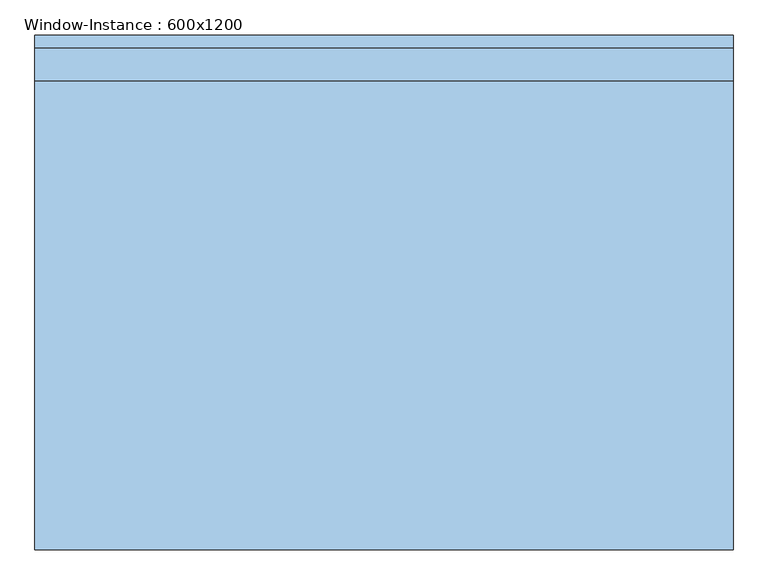
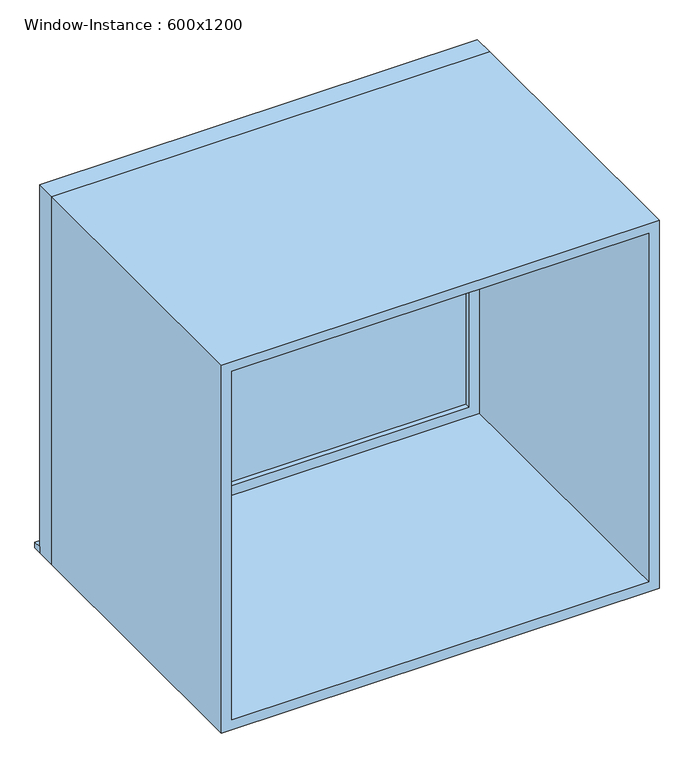
"""IFC4 building model written with IfcOpenShell, lengths in millimetres: window geometry, Window-Instance : 600x1200."""

from ifc_helpers import new_model, si_unit, frame, origin, place, context, project, spatial, polyline, outline, extrude, source, transform, mapped, element, save


def window_instance_600x1200_9ff07a73(model_context):
    return source(origin(), model_context, "Body", "SweptSolid", [
        extrude(outline(polyline([(-713.1, 510.4), (636.9, 510.4), (636.9, 485.0), (-713.1, 485.0), (-713.1, 510.4)])), frame((0.0, 0.0, 900.0), z_axis=(0.0, 0.0, 1.0), x_axis=(1.0, 0.0, 0.0)), (0.0, 0.0, 1.0), 19.05),
        extrude(outline(polyline([(573.4, 436.425), (-649.6, 436.425), (-649.6, 449.125), (573.4, 449.125), (573.4, 436.425)])), frame((0.0, 0.0, 963.5), z_axis=(0.0, 0.0, 1.0), x_axis=(1.0, 0.0, 0.0)), (0.0, 0.0, 1.0), 1073.0),
        extrude(outline(polyline([(2080.95, -694.05), (919.05, -694.05), (919.05, 617.85), (2080.95, 617.85), (2080.95, -694.05)]), holes=[polyline([(2036.5, -649.6), (2036.5, 573.4), (963.5, 573.4), (963.5, -649.6), (2036.5, -649.6)])]), frame((0.0, 420.55, 0.0), z_axis=(0.0, 1.0, 0.0), x_axis=(0.0, 0.0, 1.0)), (0.0, 0.0, 1.0), 44.45),
        extrude(outline(polyline([(2100.0, -713.1), (900.0, -713.1), (900.0, 636.9), (2100.0, 636.9), (2100.0, -713.1)]), holes=[polyline([(2068.25, -681.35), (2068.25, 605.15), (931.75, 605.15), (931.75, -681.35), (2068.25, -681.35)])]), frame((0.0, -485.0, 0.0), z_axis=(0.0, 1.0, 0.0), x_axis=(0.0, 0.0, 1.0)), (0.0, 0.0, 1.0), 905.55),
        extrude(outline(polyline([(2100.0, 636.9), (2100.0, -713.1), (900.0, -713.1), (900.0, 636.9), (2100.0, 636.9)]), holes=[polyline([(2080.95, 617.85), (919.05, 617.85), (919.05, -694.05), (2080.95, -694.05), (2080.95, 617.85)])]), frame((0.0, 420.55, 0.0), z_axis=(0.0, 1.0, 0.0), x_axis=(0.0, 0.0, 1.0)), (0.0, 0.0, 1.0), 64.45),
    ])


if __name__ == "__main__":
    model = new_model("IFC4")
    model_context = context("Model", 3, world=origin())
    ifc_project = project(units=[si_unit("LENGTHUNIT", "METRE", prefix="MILLI")], contexts=[model_context])
    site = spatial("IfcSite", under=ifc_project)
    building = spatial("IfcBuilding", under=site)
    placement = place(None, origin())
    window_instance_600x1200_shape = window_instance_600x1200_9ff07a73(model_context)
    element("IfcWindow", 1, ObjectType="Window-Instance : 600x1200", at=placement, inside=building, context=model_context, shape_type="MappedRepresentation", body=[
        mapped(window_instance_600x1200_shape, transform((0.0, 0.0, 0.0), x_axis=(1.0, 0.0, 0.0), y_axis=(0.0, 1.0, 0.0), z_axis=(0.0, 0.0, 1.0))),
    ])
    save(model, "model.ifc")

# Revit data of these elements
# Type "Window-Instance : 600x1200"
#   Type Mark = "7"
#   Construction Type Id = "GSP4R"
#   Assembly Code = "B2020100"
#   Analytic Construction = "1/8 in Pilkington single glazing"
#   Visual Light Transmittance = 0.9
#   Thermal Resistance (R) = 0.149095 (m²·K)/W
#   Solar Heat Gain Coefficient = 0.86
#   Heat Transfer Coefficient (U) = 6.70716 W/(m²·K)
#   Height [instance default] = 1200 mm
#   Default Sill Height = 900 mm
#   Width [instance default] = 600 mm
#   Window Inset = 20 mm
#   Glass Pane Material = WW-EC-GL-Storefront
#   Sash Material = WW-EC-RGB-White
#   Wall Closure = (empty or 0)
# Element 1 (IfcWindow, "Window-Instance : 600x1200")
#   Width = 1350 mm
#   Materials on its faces: "WW-EC-RGB-White", "WW-EC-GL-Storefront"
# Materials
#   "WW-EC-GL-Storefront": class "Glass", colour RGB 236 240 239, transparency 0.85, Description = "Storefront Glass", Cost = 0
#   "WW-EC-RGB-White": class "Generic", colour RGB 255 255 255, transparency 0, Comments = "If region requests off-white, swith asset color to RGB 231-228-220", Description = "Generic Color", Cost = 0
